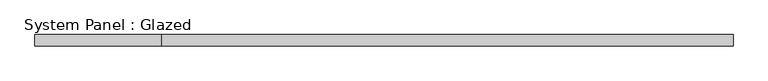
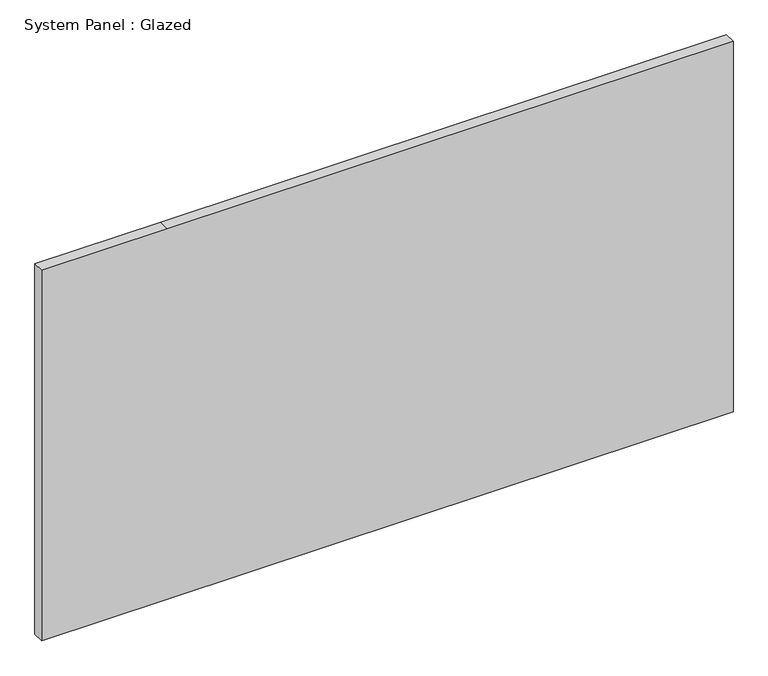
"""IFC4 building model written with IfcOpenShell, lengths in millimetres: plate geometry, System Panel : Glazed."""

from ifc_helpers import new_model, si_unit, frame, origin, place, context, project, spatial, polyline, outline, extrude, source, transform, mapped, element, save


def system_panel_glazed_de38c793(model_context):
    return source(origin(), model_context, "Body", "SweptSolid", [
        extrude(outline(polyline([(0.0, -768.35), (0.0, -488.95), (0.0, 768.35), (869.95, 768.35), (869.95, -488.95), (869.95, -768.35), (0.0, -768.35)])), frame((0.0, -44.45, 0.0), z_axis=(0.0, 1.0, 0.0), x_axis=(0.0, 0.0, 1.0)), (0.0, 0.0, 1.0), 25.4),
    ])


if __name__ == "__main__":
    model = new_model("IFC4")
    model_context = context("Model", 3, world=origin())
    ifc_project = project(units=[si_unit("LENGTHUNIT", "METRE", prefix="MILLI")], contexts=[model_context])
    site = spatial("IfcSite", under=ifc_project)
    building = spatial("IfcBuilding", under=site)
    placement = place(None, origin())
    system_panel_glazed_shape = system_panel_glazed_de38c793(model_context)
    element("IfcPlate", 1, ObjectType="System Panel : Glazed", at=placement, inside=building, context=model_context, shape_type="MappedRepresentation", body=[
        mapped(system_panel_glazed_shape, transform((0.0, 0.0, 0.0), x_axis=(1.0, 0.0, 0.0), y_axis=(0.0, 1.0, 0.0), z_axis=(0.0, 0.0, 1.0))),
    ])
    save(model, "model.ifc")

# Revit data of these elements
# Element 1 (IfcPlate, "System Panel : Glazed")
#   Materials on its faces: "Glass"
# Materials
#   "Glass": class "Glass", colour RGB 0 128 192, transparency 0.75
